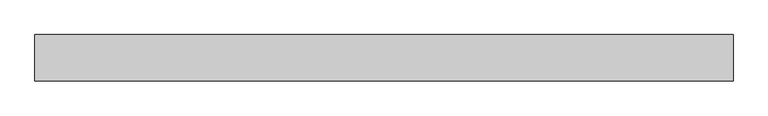
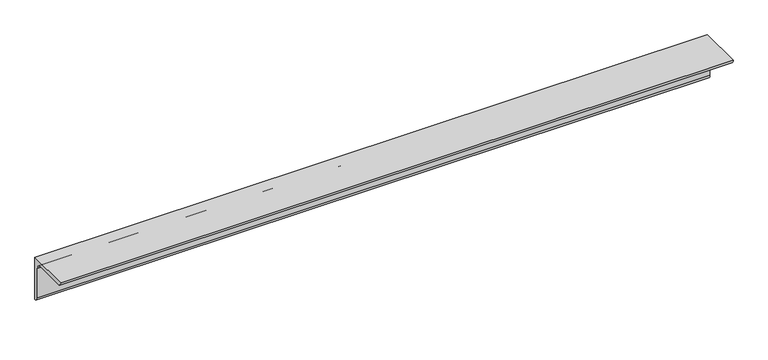
"""IFC4 building model written with IfcOpenShell, lengths in millimetres: member geometry, 0912_Steel Framing_L-KSD3502 : H_SB_AR_S04_L-100x100x10_KBR2."""

import ifcopenshell
import ifcopenshell.guid

model = None  # the IFC model being written
_history = None  # IfcOwnerHistory: only IFC2X3 demands one
_inside = {}  # id of a spatial element -> (the spatial element, [elements in it])
_under = {}  # id of a project, library or spatial element -> (it, [spatial elements below it])
_declared = {}  # id of a project -> (the project, [libraries it declares])
_typed = {}  # id of a type object -> (the type object, [elements of that type])
_made_of = {}  # id of a material, layer set ... -> (it, [elements and type objects made of it])


def new_model(schema):
    """Start an empty IFC model of exactly this schema.

    Asked for "IFC4X3", IfcOpenShell would pick the latest addendum, in which some entities
    have other attributes; the version numbers below select the first issue.
    IFC2X3 requires an IfcOwnerHistory on every rooted entity: one is made here for all.
    """
    global model, _history
    if schema == "IFC4X3":
        model = ifcopenshell.file(schema_version=(4, 3, 0, 0))
    else:
        model = ifcopenshell.file(schema=schema)
    _inside.clear()
    _under.clear()
    _declared.clear()
    _typed.clear()
    _made_of.clear()
    _history = None
    if model.schema == "IFC2X3":
        org = make("IfcOrganization", Name="unknown")
        user = make(
            "IfcPersonAndOrganization",
            ThePerson=make("IfcPerson", FamilyName="unknown"),
            TheOrganization=org,
        )
        app = make(
            "IfcApplication",
            ApplicationDeveloper=org,
            Version="unknown",
            ApplicationFullName="unknown",
            ApplicationIdentifier="unknown",
        )
        _history = make(
            "IfcOwnerHistory",
            OwningUser=user,
            OwningApplication=app,
            ChangeAction="ADDED",
            CreationDate=0,
        )
    return model


def make(cls, **values):
    """One entity of the class cls with the attributes given. An attribute that is None is left unset."""
    return model.create_entity(
        cls, **{name: value for name, value in values.items() if value is not None}
    )


def rooted(cls, **values):
    """An entity with a GlobalId (a new one), such as an element, a storey or a relation."""
    return make(cls, GlobalId=ifcopenshell.guid.new(), OwnerHistory=_history, **values)


def si_unit(unit_type, name, prefix=None):
    """IfcSIUnit, for example si_unit("LENGTHUNIT", "METRE", prefix="MILLI")."""
    return make("IfcSIUnit", UnitType=unit_type, Prefix=prefix, Name=name)


def assignment(units):
    """IfcUnitAssignment: the units of a project."""
    return None if units is None else make("IfcUnitAssignment", Units=units)


def point(xyz):
    """IfcCartesianPoint."""
    return None if xyz is None else make("IfcCartesianPoint", Coordinates=xyz)


def direction(xyz):
    """IfcDirection."""
    return None if xyz is None else make("IfcDirection", DirectionRatios=xyz)


def frame(location, z_axis=None, x_axis=None):
    """IfcAxis2Placement3D, a coordinate frame: its origin and axes. An axis left out is left unset."""
    return make(
        "IfcAxis2Placement3D",
        Location=point(location),
        Axis=direction(z_axis),
        RefDirection=direction(x_axis),
    )


def frame_2d(location, x_axis=None):
    """IfcAxis2Placement2D, a coordinate frame in the plane: its origin and x axis."""
    return make(
        "IfcAxis2Placement2D", Location=point(location), RefDirection=direction(x_axis)
    )


def origin():
    """The frame at (0, 0, 0) with its axes left unset."""
    return frame((0.0, 0.0, 0.0))


def place(relative_to, where):
    """IfcLocalPlacement: puts the frame where relative to a parent placement (None: the world)."""
    return make(
        "IfcLocalPlacement", PlacementRelTo=relative_to, RelativePlacement=where
    )


def context(
    kind, dimensions, precision=None, world=None, true_north=None, identifier=None
):
    """IfcGeometricRepresentationContext, for example the 3D "Model" context."""
    return make(
        "IfcGeometricRepresentationContext",
        ContextIdentifier=identifier,
        ContextType=kind,
        CoordinateSpaceDimension=dimensions,
        Precision=precision,
        WorldCoordinateSystem=world,
        TrueNorth=true_north,
    )


def project(units=None, contexts=None):
    """IfcProject with its units and contexts."""
    return rooted(
        "IfcProject",
        Name="project",
        RepresentationContexts=contexts,
        UnitsInContext=assignment(units),
    )


def spatial(cls, under=None, at=None, **own):
    """A site, building, storey or space (cls), placed at a placement, below another one or the project."""
    s = rooted(cls, ObjectPlacement=at, **own)
    if under is not None:
        _under.setdefault(under.id(), (under, []))[1].append(s)
    return s


def polyline(points):
    """IfcPolyline through the points."""
    return make("IfcPolyline", Points=[point(p) for p in points])


def circle_curve(where, radius):
    """IfcCircle in the frame where."""
    return make("IfcCircle", Position=where, Radius=radius)


def trimmed(basis, trim1, trim2, sense, master):
    """IfcTrimmedCurve: the piece of a basis curve between two trims."""
    return make(
        "IfcTrimmedCurve",
        BasisCurve=basis,
        Trim1=trim1,
        Trim2=trim2,
        SenseAgreement=sense,
        MasterRepresentation=master,
    )


def segment(curve, same_sense, transition):
    """IfcCompositeCurveSegment."""
    return make(
        "IfcCompositeCurveSegment",
        Transition=transition,
        SameSense=same_sense,
        ParentCurve=curve,
    )


def composite_curve(segments, self_intersect=None):
    """IfcCompositeCurve: segments joined end to end."""
    return make("IfcCompositeCurve", Segments=segments, SelfIntersect=self_intersect)


def outline(outer, holes=None, kind="AREA"):
    """IfcArbitraryClosedProfileDef: a profile drawn as a closed curve; with holes, ...WithVoids."""
    if holes is None:
        return make("IfcArbitraryClosedProfileDef", ProfileType=kind, OuterCurve=outer)
    return make(
        "IfcArbitraryProfileDefWithVoids",
        ProfileType=kind,
        OuterCurve=outer,
        InnerCurves=holes,
    )


def extrude(swept, where, along, depth):
    """IfcExtrudedAreaSolid: the profile swept, set in the frame where, extruded along a direction by depth."""
    return make(
        "IfcExtrudedAreaSolid",
        SweptArea=swept,
        Position=where,
        ExtrudedDirection=direction(along),
        Depth=depth,
    )


def shape(context_of_items, identifier, shape_type, items):
    """IfcShapeRepresentation: the items that make up one representation, for example the "Body"."""
    return make(
        "IfcShapeRepresentation",
        ContextOfItems=context_of_items,
        RepresentationIdentifier=identifier,
        RepresentationType=shape_type,
        Items=items,
    )


def source(mapping_origin, context_of_items, identifier, shape_type, items):
    """IfcRepresentationMap: a shape defined once, which mapped items show again and again."""
    return make(
        "IfcRepresentationMap",
        MappingOrigin=mapping_origin,
        MappedRepresentation=shape(context_of_items, identifier, shape_type, items),
    )


def transform(
    local_origin,
    x_axis=None,
    y_axis=None,
    z_axis=None,
    scale=None,
    scale2=None,
    scale3=None,
    uniform=True,
):
    """IfcCartesianTransformationOperator3D, or its non-uniform kind. x_axis, y_axis, z_axis: its Axis1, 2, 3."""
    if uniform:
        return make(
            "IfcCartesianTransformationOperator3D",
            Axis1=direction(x_axis),
            Axis2=direction(y_axis),
            LocalOrigin=point(local_origin),
            Scale=scale,
            Axis3=direction(z_axis),
        )
    return make(
        "IfcCartesianTransformationOperator3DnonUniform",
        Axis1=direction(x_axis),
        Axis2=direction(y_axis),
        LocalOrigin=point(local_origin),
        Scale=scale,
        Axis3=direction(z_axis),
        Scale2=scale2,
        Scale3=scale3,
    )


def mapped(mapping_source, mapping_target):
    """IfcMappedItem: shows the shape of a source again, moved by a transform."""
    return make(
        "IfcMappedItem", MappingSource=mapping_source, MappingTarget=mapping_target
    )


def made_of(thing, what):
    """Note that an element or type object is made of a material, layer set ...; save() writes the relation."""
    if what is not None:
        _made_of.setdefault(what.id(), (what, []))[1].append(thing)
    return thing


def element(
    cls,
    number,
    at=None,
    inside=None,
    cuts=None,
    type_object=None,
    material=None,
    context=None,
    identifier="Body",
    shape_type=None,
    held_by="IfcProductDefinitionShape",
    body=None,
    shapes=None,
    **own,
):
    """One element of the class cls, such as IfcWall. Its Tag is "e" and its number.

    at: its placement. inside: the storey or other place that contains it. cuts: it is an
    opening in that element (IfcRelVoidsElement). A single representation is given by context,
    identifier, shape_type and body (its items); several are given by shapes. held_by: the class
    of the entity that holds the representations. save() writes the other relations.
    """
    e = rooted(cls, Tag="e%d" % number, ObjectPlacement=at, **own)
    if body is not None:
        shapes = [shape(context, identifier, shape_type, body)]
    if shapes is not None:
        e.Representation = make(held_by, Representations=shapes)
    if inside is not None:
        _inside.setdefault(inside.id(), (inside, []))[1].append(e)
    if cuts is not None:
        rooted(
            "IfcRelVoidsElement", RelatingBuildingElement=cuts, RelatedOpeningElement=e
        )
    if type_object is not None:
        _typed.setdefault(type_object.id(), (type_object, []))[1].append(e)
    return made_of(e, material)


def aggregate(whole, parts):
    """IfcRelAggregates: a whole, such as a stair, and the parts it consists of."""
    return rooted("IfcRelAggregates", RelatingObject=whole, RelatedObjects=parts)


def save(model, path):
    """Write the relations noted so far, then the file.

    IfcRelAggregates (storeys below a building ...), IfcRelContainedInSpatialStructure (elements
    in a storey), IfcRelDefinesByType, IfcRelAssociatesMaterial and IfcRelDeclares: one each for
    every whole, place, type object, material and project.
    """
    for whole, parts in _under.values():
        aggregate(whole, parts)
    for where, things in _inside.values():
        rooted(
            "IfcRelContainedInSpatialStructure",
            RelatedElements=things,
            RelatingStructure=where,
        )
    for kind, things in _typed.values():
        rooted("IfcRelDefinesByType", RelatedObjects=things, RelatingType=kind)
    for what, things in _made_of.values():
        rooted("IfcRelAssociatesMaterial", RelatedObjects=things, RelatingMaterial=what)
    for by, libraries in _declared.values():
        rooted("IfcRelDeclares", RelatingContext=by, RelatedDefinitions=libraries)
    model.write(path)


def member_c56ac2bd(model_context):
    return source(origin(), model_context, "Body", "SweptSolid", [
        extrude(outline(composite_curve([segment(polyline([(28.2, 28.2), (28.2, -71.8)]), True, "CONTINUOUS"), segment(trimmed(circle_curve(frame_2d((28.2, -61.8)), 10.0), [point((28.2, -71.8))], [point((18.2, -61.8))], False, "CARTESIAN"), True, "CONTINUOUS"), segment(polyline([(18.2, -61.8), (18.2, 8.2)]), True, "CONTINUOUS"), segment(trimmed(circle_curve(frame_2d((8.2, 8.2)), 10.0), [point((18.2, 8.2))], [point((8.2, 18.2))], True, "CARTESIAN"), True, "CONTINUOUS"), segment(polyline([(8.2, 18.2), (-61.8, 18.2)]), True, "CONTINUOUS"), segment(trimmed(circle_curve(frame_2d((-61.8, 28.2)), 10.0), [point((-61.8, 18.2))], [point((-71.8, 28.2))], False, "CARTESIAN"), True, "CONTINUOUS"), segment(polyline([(-71.8, 28.2), (28.2, 28.2)]), True, "CONTINUOUS")], self_intersect=False)), frame((-835.5368795, 0.0, 0.0), z_axis=(1.0, 0.0, 0.0), x_axis=(0.0, 1.0, 0.0)), (0.0, 0.0, 1.0), 1509.087639),
    ])


if __name__ == "__main__":
    model = new_model("IFC4")
    model_context = context("Model", 3, world=origin())
    ifc_project = project(units=[si_unit("LENGTHUNIT", "METRE", prefix="MILLI")], contexts=[model_context])
    site = spatial("IfcSite", under=ifc_project)
    building = spatial("IfcBuilding", under=site)
    placement = place(None, origin())
    member_shape = member_c56ac2bd(model_context)
    element("IfcMember", 1, ObjectType="0912_Steel Framing_L-KSD3502 : H_SB_AR_S04_L-100x100x10_KBR2", at=placement, inside=building, context=model_context, shape_type="MappedRepresentation", body=[
        mapped(member_shape, transform((0.0, 0.0, 0.0), x_axis=(1.0, 0.0, 0.0), y_axis=(0.0, 1.0, 0.0), z_axis=(0.0, 0.0, 1.0))),
    ])
    save(model, "model.ifc")

# Revit data of these elements
# Type "0912_Steel Framing_L-KSD3502 : H_SB_AR_S04_L-100x100x10_KBR2"
#   k = 25 mm
#   Perimeter = 0.40 m²/m
#   Nominal Weight = 14.90 kgf/m
#   Length [instance default] = 1000 mm
#   b = 100 mm
#   d = 100 mm
#   t = 10 mm
#   x = 28.2 mm
#   y = 28.2 mm
#   A = 1900.00 m²
#   Structural Material [instance default] = Steel, 45-345
# Element 1 (IfcMember, "0912_Steel Framing_L-KSD3502 : H_SB_AR_S04_L-100x100x10_KBR2")
#   Materials on its faces: "Steel, 45-345"
# Materials
#   "Steel, 45-345": class "Metal", colour RGB 189 187 185, transparency 0, Description = "Steel 345 MPa", Cost = 0
